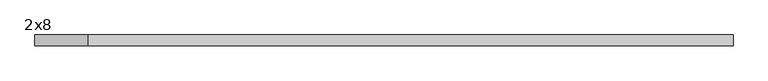
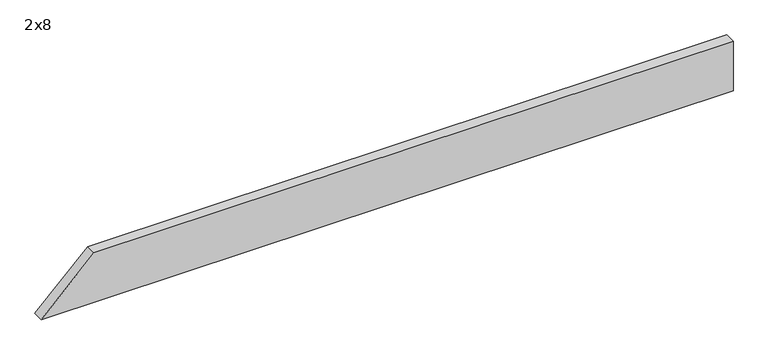
"""IFC4 building model written with IfcOpenShell, lengths in millimetres: beam geometry, Dimension Lumber - Canted Ends : 2x8."""

import ifcopenshell
import ifcopenshell.guid

model = None  # the IFC model being written
_history = None  # IfcOwnerHistory: only IFC2X3 demands one
_inside = {}  # id of a spatial element -> (the spatial element, [elements in it])
_under = {}  # id of a project, library or spatial element -> (it, [spatial elements below it])
_declared = {}  # id of a project -> (the project, [libraries it declares])
_typed = {}  # id of a type object -> (the type object, [elements of that type])
_made_of = {}  # id of a material, layer set ... -> (it, [elements and type objects made of it])


def new_model(schema):
    """Start an empty IFC model of exactly this schema.

    Asked for "IFC4X3", IfcOpenShell would pick the latest addendum, in which some entities
    have other attributes; the version numbers below select the first issue.
    IFC2X3 requires an IfcOwnerHistory on every rooted entity: one is made here for all.
    """
    global model, _history
    if schema == "IFC4X3":
        model = ifcopenshell.file(schema_version=(4, 3, 0, 0))
    else:
        model = ifcopenshell.file(schema=schema)
    _inside.clear()
    _under.clear()
    _declared.clear()
    _typed.clear()
    _made_of.clear()
    _history = None
    if model.schema == "IFC2X3":
        org = make("IfcOrganization", Name="unknown")
        user = make(
            "IfcPersonAndOrganization",
            ThePerson=make("IfcPerson", FamilyName="unknown"),
            TheOrganization=org,
        )
        app = make(
            "IfcApplication",
            ApplicationDeveloper=org,
            Version="unknown",
            ApplicationFullName="unknown",
            ApplicationIdentifier="unknown",
        )
        _history = make(
            "IfcOwnerHistory",
            OwningUser=user,
            OwningApplication=app,
            ChangeAction="ADDED",
            CreationDate=0,
        )
    return model


def make(cls, **values):
    """One entity of the class cls with the attributes given. An attribute that is None is left unset."""
    return model.create_entity(
        cls, **{name: value for name, value in values.items() if value is not None}
    )


def rooted(cls, **values):
    """An entity with a GlobalId (a new one), such as an element, a storey or a relation."""
    return make(cls, GlobalId=ifcopenshell.guid.new(), OwnerHistory=_history, **values)


def si_unit(unit_type, name, prefix=None):
    """IfcSIUnit, for example si_unit("LENGTHUNIT", "METRE", prefix="MILLI")."""
    return make("IfcSIUnit", UnitType=unit_type, Prefix=prefix, Name=name)


def assignment(units):
    """IfcUnitAssignment: the units of a project."""
    return None if units is None else make("IfcUnitAssignment", Units=units)


def point(xyz):
    """IfcCartesianPoint."""
    return None if xyz is None else make("IfcCartesianPoint", Coordinates=xyz)


def direction(xyz):
    """IfcDirection."""
    return None if xyz is None else make("IfcDirection", DirectionRatios=xyz)


def frame(location, z_axis=None, x_axis=None):
    """IfcAxis2Placement3D, a coordinate frame: its origin and axes. An axis left out is left unset."""
    return make(
        "IfcAxis2Placement3D",
        Location=point(location),
        Axis=direction(z_axis),
        RefDirection=direction(x_axis),
    )


def origin():
    """The frame at (0, 0, 0) with its axes left unset."""
    return frame((0.0, 0.0, 0.0))


def place(relative_to, where):
    """IfcLocalPlacement: puts the frame where relative to a parent placement (None: the world)."""
    return make(
        "IfcLocalPlacement", PlacementRelTo=relative_to, RelativePlacement=where
    )


def context(
    kind, dimensions, precision=None, world=None, true_north=None, identifier=None
):
    """IfcGeometricRepresentationContext, for example the 3D "Model" context."""
    return make(
        "IfcGeometricRepresentationContext",
        ContextIdentifier=identifier,
        ContextType=kind,
        CoordinateSpaceDimension=dimensions,
        Precision=precision,
        WorldCoordinateSystem=world,
        TrueNorth=true_north,
    )


def project(units=None, contexts=None):
    """IfcProject with its units and contexts."""
    return rooted(
        "IfcProject",
        Name="project",
        RepresentationContexts=contexts,
        UnitsInContext=assignment(units),
    )


def spatial(cls, under=None, at=None, **own):
    """A site, building, storey or space (cls), placed at a placement, below another one or the project."""
    s = rooted(cls, ObjectPlacement=at, **own)
    if under is not None:
        _under.setdefault(under.id(), (under, []))[1].append(s)
    return s


def polyline(points):
    """IfcPolyline through the points."""
    return make("IfcPolyline", Points=[point(p) for p in points])


def outline(outer, holes=None, kind="AREA"):
    """IfcArbitraryClosedProfileDef: a profile drawn as a closed curve; with holes, ...WithVoids."""
    if holes is None:
        return make("IfcArbitraryClosedProfileDef", ProfileType=kind, OuterCurve=outer)
    return make(
        "IfcArbitraryProfileDefWithVoids",
        ProfileType=kind,
        OuterCurve=outer,
        InnerCurves=holes,
    )


def extrude(swept, where, along, depth):
    """IfcExtrudedAreaSolid: the profile swept, set in the frame where, extruded along a direction by depth."""
    return make(
        "IfcExtrudedAreaSolid",
        SweptArea=swept,
        Position=where,
        ExtrudedDirection=direction(along),
        Depth=depth,
    )


def shape(context_of_items, identifier, shape_type, items):
    """IfcShapeRepresentation: the items that make up one representation, for example the "Body"."""
    return make(
        "IfcShapeRepresentation",
        ContextOfItems=context_of_items,
        RepresentationIdentifier=identifier,
        RepresentationType=shape_type,
        Items=items,
    )


def source(mapping_origin, context_of_items, identifier, shape_type, items):
    """IfcRepresentationMap: a shape defined once, which mapped items show again and again."""
    return make(
        "IfcRepresentationMap",
        MappingOrigin=mapping_origin,
        MappedRepresentation=shape(context_of_items, identifier, shape_type, items),
    )


def transform(
    local_origin,
    x_axis=None,
    y_axis=None,
    z_axis=None,
    scale=None,
    scale2=None,
    scale3=None,
    uniform=True,
):
    """IfcCartesianTransformationOperator3D, or its non-uniform kind. x_axis, y_axis, z_axis: its Axis1, 2, 3."""
    if uniform:
        return make(
            "IfcCartesianTransformationOperator3D",
            Axis1=direction(x_axis),
            Axis2=direction(y_axis),
            LocalOrigin=point(local_origin),
            Scale=scale,
            Axis3=direction(z_axis),
        )
    return make(
        "IfcCartesianTransformationOperator3DnonUniform",
        Axis1=direction(x_axis),
        Axis2=direction(y_axis),
        LocalOrigin=point(local_origin),
        Scale=scale,
        Axis3=direction(z_axis),
        Scale2=scale2,
        Scale3=scale3,
    )


def mapped(mapping_source, mapping_target):
    """IfcMappedItem: shows the shape of a source again, moved by a transform."""
    return make(
        "IfcMappedItem", MappingSource=mapping_source, MappingTarget=mapping_target
    )


def made_of(thing, what):
    """Note that an element or type object is made of a material, layer set ...; save() writes the relation."""
    if what is not None:
        _made_of.setdefault(what.id(), (what, []))[1].append(thing)
    return thing


def element(
    cls,
    number,
    at=None,
    inside=None,
    cuts=None,
    type_object=None,
    material=None,
    context=None,
    identifier="Body",
    shape_type=None,
    held_by="IfcProductDefinitionShape",
    body=None,
    shapes=None,
    **own,
):
    """One element of the class cls, such as IfcWall. Its Tag is "e" and its number.

    at: its placement. inside: the storey or other place that contains it. cuts: it is an
    opening in that element (IfcRelVoidsElement). A single representation is given by context,
    identifier, shape_type and body (its items); several are given by shapes. held_by: the class
    of the entity that holds the representations. save() writes the other relations.
    """
    e = rooted(cls, Tag="e%d" % number, ObjectPlacement=at, **own)
    if body is not None:
        shapes = [shape(context, identifier, shape_type, body)]
    if shapes is not None:
        e.Representation = make(held_by, Representations=shapes)
    if inside is not None:
        _inside.setdefault(inside.id(), (inside, []))[1].append(e)
    if cuts is not None:
        rooted(
            "IfcRelVoidsElement", RelatingBuildingElement=cuts, RelatedOpeningElement=e
        )
    if type_object is not None:
        _typed.setdefault(type_object.id(), (type_object, []))[1].append(e)
    return made_of(e, material)


def aggregate(whole, parts):
    """IfcRelAggregates: a whole, such as a stair, and the parts it consists of."""
    return rooted("IfcRelAggregates", RelatingObject=whole, RelatedObjects=parts)


def save(model, path):
    """Write the relations noted so far, then the file.

    IfcRelAggregates (storeys below a building ...), IfcRelContainedInSpatialStructure (elements
    in a storey), IfcRelDefinesByType, IfcRelAssociatesMaterial and IfcRelDeclares: one each for
    every whole, place, type object, material and project.
    """
    for whole, parts in _under.values():
        aggregate(whole, parts)
    for where, things in _inside.values():
        rooted(
            "IfcRelContainedInSpatialStructure",
            RelatedElements=things,
            RelatingStructure=where,
        )
    for kind, things in _typed.values():
        rooted("IfcRelDefinesByType", RelatedObjects=things, RelatingType=kind)
    for what, things in _made_of.values():
        rooted("IfcRelAssociatesMaterial", RelatedObjects=things, RelatingMaterial=what)
    for by, libraries in _declared.values():
        rooted("IfcRelDeclares", RelatingContext=by, RelatedDefinitions=libraries)
    model.write(path)


def beam_2x8_da07914c(model_context):
    return source(origin(), model_context, "Body", "SweptSolid", [
        extrude(outline(polyline([(-92.075, -1219.2), (-92.075, 1219.2), (92.075, 1219.2), (92.075, -1033.0502844), (-92.075, -1219.2)])), frame((0.0, -19.05, 0.0), z_axis=(0.0, 1.0, 0.0), x_axis=(0.0, 0.0, 1.0)), (0.0, 0.0, 1.0), 38.1),
    ])


if __name__ == "__main__":
    model = new_model("IFC4")
    model_context = context("Model", 3, world=origin())
    ifc_project = project(units=[si_unit("LENGTHUNIT", "METRE", prefix="MILLI")], contexts=[model_context])
    site = spatial("IfcSite", under=ifc_project)
    building = spatial("IfcBuilding", under=site)
    placement = place(None, origin())
    beam_2x8_shape = beam_2x8_da07914c(model_context)
    element("IfcBeam", 1, ObjectType="Dimension Lumber - Canted Ends : 2x8", at=placement, inside=building, context=model_context, shape_type="MappedRepresentation", body=[
        mapped(beam_2x8_shape, transform((0.0, 0.0, 0.0), x_axis=(1.0, 0.0, 0.0), y_axis=(0.0, 1.0, 0.0), z_axis=(0.0, 0.0, 1.0))),
    ])
    save(model, "model.ifc")

# Revit data of these elements
# Type "Dimension Lumber - Canted Ends : 2x8"
#   Assembly Code = "B10"
#   Angle_End = 0.00°
#   Angle_Start = 45.3094°
#   A = 0.0755556 SF
#   Length [instance default] = 5' - 0"
#   b = 0' - 1 1/2"
#   d = 0' - 7 1/4"
#   Structural Material = PRE-ENGINEERED TRUSS @ 24" O.C.
# Element 1 (IfcBeam, "Dimension Lumber - Canted Ends : 2x8")
#   Materials on its faces: "PRE-ENGINEERED TRUSS @ 24\" O.C."
# Materials
#   "PRE-ENGINEERED TRUSS @ 24\" O.C.": class "Wood", colour RGB 255 255 255, transparency 0, Description = "Pinus Echinata", Cost = 0
